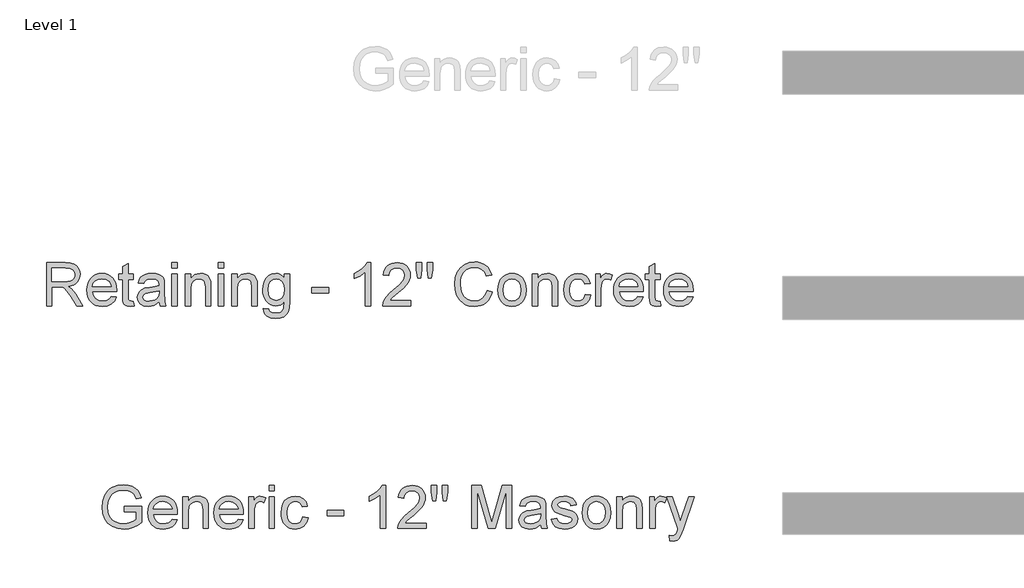
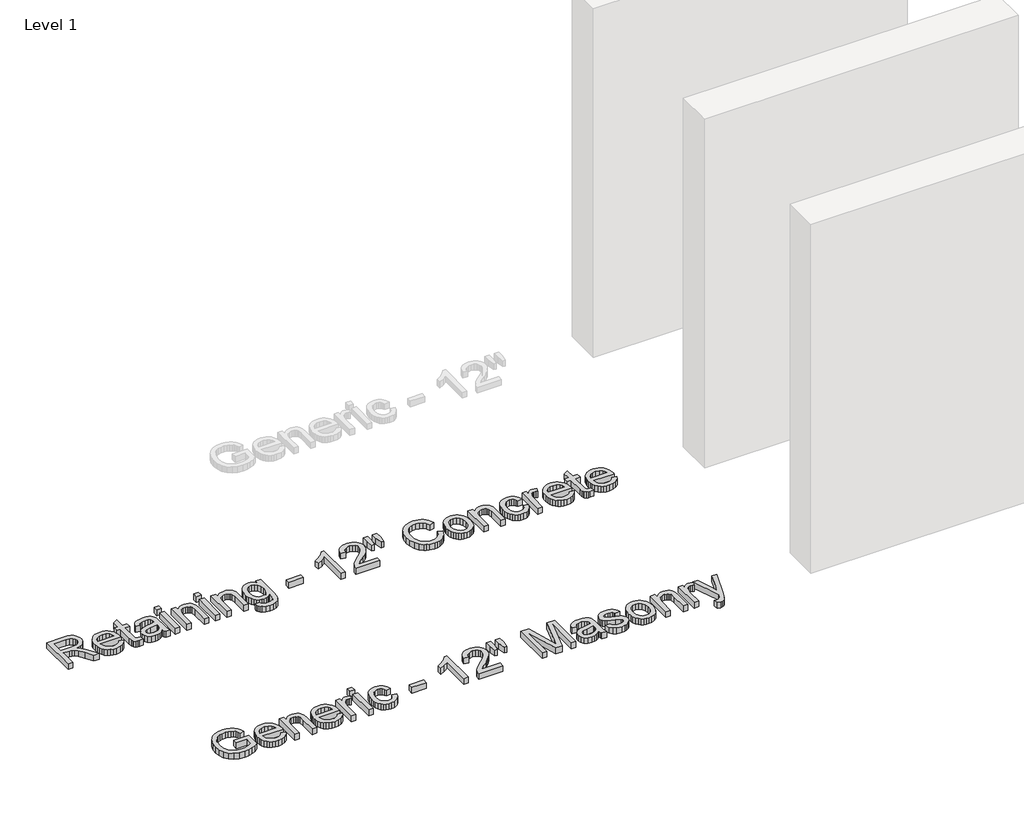
# One storey, part 19 of 42: 2 proxies.
"""IFC4 building model written with IfcOpenShell, lengths in millimetres."""

from ifc_helpers import new_model, si_unit, origin, origin_with_axes, place, context, project, spatial, polyline, outline, extrude, element, save

model = new_model("IFC4")

# Units and contexts
model_context = context("Model", 3, world=origin())
ifc_project = project(units=[si_unit("LENGTHUNIT", "METRE", prefix="MILLI")], contexts=[model_context])

# Site, building, storey
site = spatial("IfcSite", under=ifc_project)
building = spatial("IfcBuilding", under=site)
storey = spatial("IfcBuildingStorey", under=building, Name="Level 1", Elevation=0.0)

# Proxies
placement = place(None, origin())
element("IfcBuildingElementProxy", 1, Name="8\" Arial", ObjectType="8\" Arial", at=placement, inside=storey, context=model_context, shape_type="SweptSolid", body=[
    extrude(outline(polyline([(-17723.2374859, 6548.4833965), (-17723.2374859, 6853.0504905), (-17591.9970266, 6853.0504905), (-17556.7238295, 6850.9963729), (-17531.0613007, 6844.8340199), (-17512.3046968, 6833.4573682), (-17497.7492747, 6815.7603544), (-17488.4081514, 6793.8156855), (-17485.2944436, 6769.6960686), (-17490.4529744, 6739.6929381), (-17505.9285668, 6714.8204544), (-17517.6514442, 6704.6846385), (-17532.1859533, 6696.584351), (-17569.6898664, 6686.490361), (-17548.051921, 6670.206134), (-17517.1936827, 6631.0198893), (-17466.4077146, 6548.4833965), (-17510.6502491, 6548.4833965), (-17550.282637, 6611.6126599), (-17578.9101593, 6653.4014067), (-17599.0237821, 6673.1432435), (-17617.1297605, 6680.3930705), (-17639.2138491, 6681.7315001), (-17685.1665991, 6681.7315001), (-17685.1665991, 6548.4833965), (-17723.2374859, 6548.4833965)]), holes=[polyline([(-17685.1665991, 6719.8023869), (-17599.9532471, 6719.8023869), (-17575.4804334, 6721.1501112), (-17556.4914633, 6725.1932839), (-17542.1962915, 6732.2014501), (-17531.8048727, 6742.4441545), (-17525.4752159, 6754.8339231), (-17523.3653304, 6768.2832817), (-17527.3899139, 6786.8539926), (-17539.4636643, 6801.8183793), (-17560.2372073, 6811.6892977), (-17590.3611682, 6814.9796038), (-17685.1665991, 6814.9796038), (-17685.1665991, 6719.8023869)])]), origin_with_axes(), (0.0, 0.0, 1.0), 50.8),
    extrude(outline(polyline([(-17266.832988, 6615.1074483), (-17229.5056732, 6610.3485875), (-17242.9550319, 6582.2229763), (-17264.4163789, 6561.1984778), (-17293.4063926, 6548.0930212), (-17329.441751, 6543.7245356), (-17353.0641041, 6545.6090259), (-17374.1118393, 6551.2624969), (-17392.5849563, 6560.6849484), (-17408.4834553, 6573.8763805), (-17421.2682465, 6590.4696546), (-17430.4002402, 6610.0976319), (-17435.8794364, 6632.7603125), (-17437.7058352, 6658.4576963), (-17435.8608471, 6685.0264536), (-17430.325883, 6708.4443245), (-17421.1009428, 6728.711309), (-17408.1860265, 6745.8274071), (-17392.3293534, 6759.4254802), (-17374.279143, 6769.1383896), (-17354.0353951, 6774.9661352), (-17331.5981098, 6776.908717), (-17309.8834835, 6774.9707825), (-17290.2462115, 6769.1569789), (-17272.6862939, 6759.4673061), (-17257.2037305, 6745.9017643), (-17244.56533, 6728.8228448), (-17235.5379011, 6708.5930389), (-17230.1214438, 6685.2123466), (-17228.315958, 6658.6807679), (-17228.5390296, 6648.4194742), (-17399.6349484, 6648.4194742), (-17393.0450415, 6619.922077), (-17377.7367528, 6598.9719358), (-17355.6433695, 6586.0895507), (-17328.6981789, 6581.7954224), (-17308.4358418, 6583.7844775), (-17291.3708642, 6589.7516429), (-17277.5032463, 6600.0687045), (-17266.832988, 6615.1074483)]), holes=[polyline([(-17399.6349484, 6686.490361), (-17266.3868448, 6686.490361), (-17271.5360809, 6706.6039838), (-17281.6300709, 6720.9921021), (-17303.8256953, 6734.3763982), (-17331.7468242, 6738.8378303), (-17357.4093531, 6735.2779793), (-17378.6290392, 6724.5984263), (-17393.3796489, 6707.951708), (-17399.6349484, 6686.490361)])]), origin_with_axes(), (0.0, 0.0, 1.0), 50.8),
    extrude(outline(polyline([(-17109.3444369, 6580.2339212), (-17104.585576, 6547.3680385), (-17133.0643839, 6543.7245356), (-17151.337666, 6545.3046261), (-17164.963623, 6550.0448977), (-17174.5928805, 6557.3504927), (-17180.876064, 6566.6265534), (-17184.3336738, 6582.5575837), (-17185.4862104, 6609.8280871), (-17185.4862104, 6734.0789694), (-17214.0393755, 6734.0789694), (-17214.0393755, 6772.1498562), (-17185.4862104, 6772.1498562), (-17185.4862104, 6826.5049699), (-17147.4153236, 6848.8864873), (-17147.4153236, 6772.1498562), (-17109.3444369, 6772.1498562), (-17109.3444369, 6734.0789694), (-17147.4153236, 6734.0789694), (-17147.4153236, 6610.9434451), (-17145.4076792, 6591.3131441), (-17138.9014242, 6584.3607458), (-17125.9260926, 6581.7954224), (-17109.3444369, 6580.2339212)])), origin_with_axes(), (0.0, 0.0, 1.0), 50.8),
    extrude(outline(polyline([(-16928.5077248, 6577.0365615), (-16946.697355, 6561.4401387), (-16965.4260749, 6551.2346129), (-16985.1214385, 6545.602055), (-17006.2109995, 6543.7245356), (-17038.0265868, 6548.2417356), (-17061.4955782, 6561.7933354), (-17075.9673484, 6582.3716907), (-17080.7912718, 6607.969157), (-17078.9695204, 6623.7514729), (-17073.5042661, 6638.0838233), (-17065.0740185, 6650.3527614), (-17054.357287, 6659.9448403), (-17027.7002305, 6672.43685), (-16994.7599906, 6678.1623545), (-16955.833996, 6684.1852878), (-16928.7307964, 6691.2492218), (-16928.5077248, 6699.7259427), (-16931.1288161, 6716.7165631), (-16938.9920901, 6727.8329646), (-16956.577568, 6736.0866138), (-16981.0782657, 6738.8378303), (-17003.7572119, 6737.0067842), (-17019.5952956, 6731.513646), (-17030.395679, 6721.3545935), (-17037.9615242, 6705.5258044), (-17076.032411, 6710.2846652), (-17069.4239148, 6731.1046814), (-17059.562291, 6747.4632656), (-17045.5273694, 6759.9738646), (-17026.3989795, 6769.2499254), (-17003.0043452, 6774.9940191), (-16976.1706904, 6776.908717), (-16950.4338043, 6775.2170907), (-16930.0320474, 6770.1422118), (-16914.6494015, 6762.511304), (-16903.9698485, 6753.1515914), (-16896.8873252, 6741.579752), (-16892.295768, 6727.3124642), (-16890.436838, 6694.0004382), (-16890.436838, 6646.6349014), (-16888.5035508, 6580.4941714), (-16880.9191163, 6548.4833965), (-16918.9900031, 6548.4833965), (-16925.0872935, 6561.7189782), (-16928.5077248, 6577.0365615)]), holes=[polyline([(-16928.5077248, 6653.1783351), (-16989.9267726, 6641.5042546), (-17022.6811195, 6635.3326069), (-17037.515381, 6625.2943848), (-17042.7203851, 6610.6460163), (-17039.8855168, 6599.3251325), (-17031.3809119, 6590.0490717), (-17017.3924636, 6583.8588347), (-16998.1060646, 6581.7954224), (-16977.6578344, 6584.0726117), (-16959.5890347, 6590.9041795), (-16944.9406661, 6600.9702855), (-16934.7537296, 6612.9510895), (-16930.2365297, 6625.2943848), (-16928.7307964, 6642.396541), (-16928.5077248, 6653.1783351)])]), origin_with_axes(), (0.0, 0.0, 1.0), 50.8),
    extrude(outline(polyline([(-16838.0893687, 6814.9796038), (-16838.0893687, 6853.0504905), (-16800.018482, 6853.0504905), (-16800.018482, 6814.9796038), (-16838.0893687, 6814.9796038)])), origin_with_axes(), (0.0, 0.0, 1.0), 50.8),
    extrude(outline(polyline([(-16838.0893687, 6548.4833965), (-16838.0893687, 6772.1498562), (-16800.018482, 6772.1498562), (-16800.018482, 6548.4833965), (-16838.0893687, 6548.4833965)])), origin_with_axes(), (0.0, 0.0, 1.0), 50.8),
    extrude(outline(polyline([(-16742.9121518, 6548.4833965), (-16742.9121518, 6772.1498562), (-16704.8412651, 6772.1498562), (-16704.8412651, 6740.9198319), (-16691.614978, 6756.6649691), (-16675.730421, 6767.9114957), (-16657.1875941, 6774.6594117), (-16635.9864972, 6776.908717), (-16617.2205987, 6775.0962603), (-16600.0347907, 6769.65889), (-16585.7024402, 6761.2751156), (-16575.4969145, 6750.6234466), (-16564.0830841, 6722.6279605), (-16562.0754397, 6685.8211462), (-16562.0754397, 6548.4833965), (-16600.1463265, 6548.4833965), (-16600.1463265, 6680.6904993), (-16604.5334013, 6714.3743112), (-16610.6028078, 6724.4032387), (-16620.0368777, 6732.1828608), (-16632.1292174, 6737.1740879), (-16646.1734337, 6738.8378303), (-16668.4712993, 6735.1013809), (-16687.4788587, 6723.8920329), (-16695.0749115, 6714.7414499), (-16700.5006635, 6702.2354982), (-16704.8412651, 6667.1574888), (-16704.8412651, 6548.4833965), (-16742.9121518, 6548.4833965)])), origin_with_axes(), (0.0, 0.0, 1.0), 50.8),
    extrude(outline(polyline([(-16509.7279704, 6814.9796038), (-16509.7279704, 6853.0504905), (-16471.6570837, 6853.0504905), (-16471.6570837, 6814.9796038), (-16509.7279704, 6814.9796038)])), origin_with_axes(), (0.0, 0.0, 1.0), 50.8),
    extrude(outline(polyline([(-16509.7279704, 6548.4833965), (-16509.7279704, 6772.1498562), (-16471.6570837, 6772.1498562), (-16471.6570837, 6548.4833965), (-16509.7279704, 6548.4833965)])), origin_with_axes(), (0.0, 0.0, 1.0), 50.8),
    extrude(outline(polyline([(-16414.5507535, 6548.4833965), (-16414.5507535, 6772.1498562), (-16376.4798668, 6772.1498562), (-16376.4798668, 6740.9198319), (-16363.2535797, 6756.6649691), (-16347.3690227, 6767.9114957), (-16328.8261958, 6774.6594117), (-16307.6250989, 6776.908717), (-16288.8592004, 6775.0962603), (-16271.6733924, 6769.65889), (-16257.341042, 6761.2751156), (-16247.1355162, 6750.6234466), (-16235.7216859, 6722.6279605), (-16233.7140414, 6685.8211462), (-16233.7140414, 6548.4833965), (-16271.7849282, 6548.4833965), (-16271.7849282, 6680.6904993), (-16276.172003, 6714.3743112), (-16282.2414095, 6724.4032387), (-16291.6754794, 6732.1828608), (-16303.7678191, 6737.1740879), (-16317.8120354, 6738.8378303), (-16340.109901, 6735.1013809), (-16359.1174604, 6723.8920329), (-16366.7135132, 6714.7414499), (-16372.1392652, 6702.2354982), (-16376.4798668, 6667.1574888), (-16376.4798668, 6548.4833965), (-16414.5507535, 6548.4833965)])), origin_with_axes(), (0.0, 0.0, 1.0), 50.8),
    extrude(outline(polyline([(-16190.8842938, 6529.4479531), (-16152.8134071, 6524.6890923), (-16148.6122252, 6512.7919401), (-16140.4701118, 6504.6126481), (-16124.4647243, 6498.2551074), (-16103.514583, 6496.1359272), (-16081.1702442, 6498.5339469), (-16064.5514098, 6505.7280061), (-16053.0260437, 6517.2533722), (-16045.9621097, 6532.6453127), (-16043.3596076, 6577.0365615), (-16056.0282157, 6564.5445518), (-16070.1653785, 6555.6216877), (-16085.771096, 6550.2679693), (-16102.8453682, 6548.4833965), (-16123.7188286, 6550.5607508), (-16142.0966755, 6556.7928137), (-16157.9789089, 6567.1795851), (-16171.3655286, 6581.7210652), (-16181.98699, 6599.1671234), (-16189.5737482, 6618.2676293), (-16194.125803, 6639.022583), (-16195.6431547, 6661.4319843), (-16192.9198222, 6692.1693922), (-16184.7498248, 6720.4344231), (-16171.4212965, 6744.3867364), (-16153.2223717, 6762.1859913), (-16130.7757917, 6773.2280356), (-16104.7042982, 6776.908717), (-16086.900396, 6774.8267154), (-16070.7416468, 6768.5807106), (-16056.2280507, 6758.1707025), (-16043.3596076, 6743.5966911), (-16043.3596076, 6772.1498562), (-16005.2887209, 6772.1498562), (-16005.2887209, 6579.044206), (-16007.8912229, 6534.4577695), (-16015.698729, 6505.0959699), (-16029.1480877, 6485.6236779), (-16048.6761475, 6470.7057645), (-16073.8553546, 6461.2252215), (-16104.258155, 6458.0650404), (-16139.6800665, 6462.5171778), (-16167.5733114, 6475.87359), (-16178.0785897, 6485.9001938), (-16185.4655128, 6498.1714556), (-16189.7340809, 6512.6873753), (-16190.8842938, 6529.4479531)]), holes=[polyline([(-16157.5722679, 6664.0344864), (-16153.5105058, 6629.114486), (-16141.3252196, 6605.1064048), (-16123.0054642, 6591.1923136), (-16100.540295, 6586.5542832), (-16078.2424294, 6591.1644297), (-16059.8297276, 6604.994869), (-16047.4771376, 6628.6962267), (-16043.3596076, 6662.9191284), (-16047.5979681, 6695.9244308), (-16060.3130494, 6719.6908511), (-16078.9952961, 6734.0510855), (-16101.1351526, 6738.8378303), (-16122.8753391, 6734.1254427), (-16141.102148, 6719.9882799), (-16153.4547379, 6696.5750563), (-16157.5722679, 6664.0344864)])]), origin_with_axes(), (0.0, 0.0, 1.0), 50.8),
    extrude(outline(polyline([(-15848.246313, 6638.9017525), (-15848.246313, 6676.9726393), (-15729.2747919, 6676.9726393), (-15729.2747919, 6638.9017525), (-15848.246313, 6638.9017525)])), origin_with_axes(), (0.0, 0.0, 1.0), 50.8),
    extrude(outline(polyline([(-15434.2254195, 6548.4833965), (-15472.2963063, 6548.4833965), (-15472.2963063, 6785.8315811), (-15508.3595486, 6760.1411683), (-15548.4380798, 6740.9198319), (-15548.4380798, 6776.908717), (-15518.5371904, 6793.1743547), (-15492.6330007, 6812.5258162), (-15472.2126544, 6833.1041715), (-15458.7632957, 6853.0504905), (-15434.2254195, 6853.0504905), (-15434.2254195, 6548.4833965)])), origin_with_axes(), (0.0, 0.0, 1.0), 50.8),
    extrude(outline(polyline([(-15148.6937688, 6586.5542832), (-15148.6937688, 6548.4833965), (-15348.5659243, 6548.4833965), (-15344.4762783, 6574.7314883), (-15335.0886817, 6595.2447811), (-15321.3511888, 6615.1446269), (-15301.479227, 6635.9739378), (-15273.6882232, 6659.2756255), (-15232.6058698, 6695.7664218), (-15207.9564578, 6722.7023177), (-15195.6317518, 6744.5633347), (-15191.5235164, 6765.8294941), (-15195.3993855, 6784.8928215), (-15207.0269928, 6800.7401999), (-15224.9006049, 6811.4197528), (-15247.5144885, 6814.9796038), (-15271.2623195, 6811.5034047), (-15289.7121999, 6801.0748073), (-15301.6186467, 6784.5117408), (-15305.7361767, 6762.6321345), (-15343.8070635, 6767.3909953), (-15340.533023, 6787.0445329), (-15334.5774759, 6804.216399), (-15325.9404223, 6818.9065934), (-15314.6218622, 6831.1151163), (-15300.8820457, 6840.7118426), (-15284.981223, 6847.566647), (-15246.6965593, 6853.0504905), (-15226.2924787, 6851.5261679), (-15208.1330561, 6846.9532001), (-15192.2182915, 6839.331587), (-15178.5481849, 6828.6613287), (-15167.5688795, 6815.7324704), (-15159.7265185, 6801.3350575), (-15155.0211019, 6785.4690898), (-15153.4526297, 6768.1345673), (-15155.144256, 6749.9263478), (-15160.2191349, 6732.0341464), (-15169.2256509, 6713.8352215), (-15182.7121881, 6694.7068317), (-15204.2107138, 6671.8698764), (-15237.2531948, 6642.5452554), (-15281.0495861, 6605.924334), (-15298.2260994, 6586.5542832), (-15148.6937688, 6586.5542832)])), origin_with_axes(), (0.0, 0.0, 1.0), 50.8),
    extrude(outline(polyline([(-15101.328232, 6743.5966911), (-15110.6228821, 6802.4132369), (-15110.6228821, 6853.0504905), (-15072.5519953, 6853.0504905), (-15072.5519953, 6802.4132369), (-15080.8800018, 6743.5966911), (-15101.328232, 6743.5966911)])), origin_with_axes(), (0.0, 0.0, 1.0), 50.8),
    extrude(outline(polyline([(-15025.4095301, 6743.5966911), (-15034.4811085, 6802.4132369), (-15034.4811085, 6853.0504905), (-14996.4102218, 6853.0504905), (-14996.4102218, 6802.4132369), (-15005.3330859, 6743.5966911), (-15025.4095301, 6743.5966911)])), origin_with_axes(), (0.0, 0.0, 1.0), 50.8),
    extrude(outline(polyline([(-14610.9424933, 6656.7474807), (-14572.8716066, 6646.9323302), (-14580.4049205, 6623.2565328), (-14590.4384953, 6602.5689653), (-14602.9723309, 6584.8696279), (-14618.0064274, 6570.1585205), (-14635.2015301, 6558.5936521), (-14654.2183842, 6550.3330318), (-14675.0569897, 6545.3766597), (-14697.7173466, 6543.7245356), (-14741.8762291, 6548.7250574), (-14760.5468575, 6554.9757096), (-14776.9449439, 6563.7266226), (-14803.825072, 6588.208731), (-14823.4181944, 6621.650882), (-14835.380409, 6660.9672518), (-14839.3678139, 6703.0720167), (-14834.8599086, 6747.4818549), (-14821.3361927, 6785.8315811), (-14799.5030597, 6816.9035964), (-14770.0669028, 6839.4803014), (-14735.1561971, 6853.2270889), (-14696.8994174, 6857.8093514), (-14675.1243759, 6856.3268547), (-14655.1571438, 6851.8793646), (-14636.9977212, 6844.4668812), (-14620.646108, 6834.0894044), (-14606.3718492, 6821.0211263), (-14594.4444894, 6805.5362393), (-14577.6304674, 6767.3166381), (-14615.7013542, 6758.2450597), (-14628.8997573, 6786.0081795), (-14646.9313785, 6805.0529175), (-14670.0192893, 6816.0670778), (-14698.3865614, 6819.7384646), (-14731.0851404, 6815.6674079), (-14757.9466791, 6803.4542377), (-14778.3298468, 6784.3816157), (-14791.5933125, 6759.7322037), (-14798.8710235, 6731.8668427), (-14801.2969271, 6703.1463739), (-14798.4248803, 6667.975418), (-14789.8087396, 6637.5633229), (-14775.1231925, 6613.0719199), (-14754.0429261, 6595.6630403), (-14728.7707725, 6585.2623269), (-14701.5095638, 6581.7954224), (-14669.7311552, 6586.5171046), (-14643.2506971, 6600.6821514), (-14623.2579047, 6624.1418482), (-14610.9424933, 6656.7474807)])), origin_with_axes(), (0.0, 0.0, 1.0), 50.8),
    extrude(outline(polyline([(-14534.8007198, 6660.3166263), (-14532.7419548, 6689.2834033), (-14526.5656599, 6714.2441861), (-14516.2718349, 6735.1989748), (-14501.8604799, 6752.1477692), (-14487.3515311, 6762.9806839), (-14471.336849, 6770.7184801), (-14453.8164336, 6775.3611578), (-14434.7902849, 6776.908717), (-14413.7866994, 6775.0242267), (-14394.7954056, 6769.3707558), (-14377.8164035, 6759.9483043), (-14362.8496932, 6746.7568721), (-14350.6341993, 6730.2426026), (-14341.9088466, 6710.8516389), (-14336.6736349, 6688.5839809), (-14334.9285644, 6663.4396288), (-14338.0143882, 6624.9783667), (-14347.2718597, 6595.7002189), (-14362.431434, 6573.7741394), (-14383.2235662, 6557.369082), (-14407.9194515, 6547.1356722), (-14434.7902849, 6543.7245356), (-14456.1005939, 6545.602055), (-14475.268486, 6551.2346129), (-14492.2939613, 6560.6222095), (-14507.1770198, 6573.7648447), (-14519.2623885, 6590.439447), (-14527.8947948, 6610.4229447), (-14533.0742386, 6633.7153378), (-14534.8007198, 6660.3166263)]), holes=[polyline([(-14496.7298331, 6660.3909835), (-14492.3241689, 6625.9357157), (-14479.1071765, 6601.3885448), (-14459.2166253, 6586.693703), (-14434.7902849, 6581.7954224), (-14410.4754803, 6586.7215869), (-14390.6221077, 6601.5000806), (-14377.4051153, 6626.3725642), (-14372.9994511, 6661.5806987), (-14377.4329992, 6695.0321444), (-14390.7336435, 6719.2447079), (-14410.6149, 6733.9395497), (-14434.7902849, 6738.8378303), (-14459.2166253, 6733.958139), (-14479.1071765, 6719.3190651), (-14492.3241689, 6694.8276621), (-14496.7298331, 6660.3909835)])]), origin_with_axes(), (0.0, 0.0, 1.0), 50.8),
    extrude(outline(polyline([(-14292.0988167, 6548.4833965), (-14292.0988167, 6772.1498562), (-14254.02793, 6772.1498562), (-14254.02793, 6740.9198319), (-14240.8016429, 6756.6649691), (-14224.9170859, 6767.9114957), (-14206.374259, 6774.6594117), (-14185.1731621, 6776.908717), (-14166.4072636, 6775.0962603), (-14149.2214556, 6769.65889), (-14134.8891052, 6761.2751156), (-14124.6835794, 6750.6234466), (-14113.2697491, 6722.6279605), (-14111.2621046, 6685.8211462), (-14111.2621046, 6548.4833965), (-14149.3329914, 6548.4833965), (-14149.3329914, 6680.6904993), (-14153.7200662, 6714.3743112), (-14159.7894728, 6724.4032387), (-14169.2235426, 6732.1828608), (-14181.3158824, 6737.1740879), (-14195.3600986, 6738.8378303), (-14217.6579642, 6735.1013809), (-14236.6655236, 6723.8920329), (-14244.2615764, 6714.7414499), (-14249.6873284, 6702.2354982), (-14254.02793, 6667.1574888), (-14254.02793, 6548.4833965), (-14292.0988167, 6548.4833965)])), origin_with_axes(), (0.0, 0.0, 1.0), 50.8),
    extrude(outline(polyline([(-13916.14881, 6629.3840308), (-13878.0779232, 6624.62517), (-13888.6924136, 6590.7647597), (-13908.6387327, 6565.176588), (-13936.0393612, 6549.0875487), (-13969.0167797, 6543.7245356), (-13990.3689146, 6545.595084), (-14009.5135701, 6551.206729), (-14026.4507463, 6560.5594706), (-14041.180443, 6573.6533089), (-14053.1031554, 6590.2419357), (-14061.6193785, 6610.0790426), (-14066.7291124, 6633.1646298), (-14068.432357, 6659.4986971), (-14065.5231316, 6693.3776967), (-14056.7954551, 6722.7394963), (-14042.109908, 6746.4501487), (-14021.3270704, 6763.3757065), (-13996.4638814, 6773.5254644), (-13969.5372801, 6776.908717), (-13937.3684962, 6772.261392), (-13911.6501994, 6758.3194169), (-13893.2003189, 6735.8263636), (-13882.8367841, 6705.5258044), (-13920.9076709, 6700.7669435), (-13927.8135959, 6717.3764832), (-13938.567506, 6729.28293), (-13952.5745437, 6736.4491052), (-13969.2398513, 6738.8378303), (-13993.8427901, 6734.1347373), (-14013.3708499, 6720.0254585), (-14026.1138152, 6695.7478325), (-14030.3614703, 6660.5396979), (-14026.2067617, 6624.8575362), (-14013.7426359, 6600.4962584), (-13994.5677728, 6586.4706314), (-13970.2808521, 6581.7954224), (-13950.5668993, 6584.7139425), (-13934.4035028, 6593.4695029), (-13922.6457704, 6608.2851751), (-13916.14881, 6629.3840308)])), origin_with_axes(), (0.0, 0.0, 1.0), 50.8),
    extrude(outline(polyline([(-13844.7658973, 6548.4833965), (-13844.7658973, 6772.1498562), (-13811.4538714, 6772.1498562), (-13811.4538714, 6739.0609019), (-13799.1477547, 6758.2450597), (-13787.8082816, 6769.5473542), (-13776.4316299, 6775.0683763), (-13764.0139774, 6776.908717), (-13745.0528912, 6773.9716076), (-13725.7943762, 6765.1602793), (-13738.5094575, 6731.0303242), (-13751.8937537, 6736.8859538), (-13765.2780498, 6738.8378303), (-13776.6454068, 6736.960311), (-13786.8044594, 6731.327753), (-13795.0116354, 6722.3677103), (-13800.5233629, 6710.5077368), (-13805.1520987, 6689.2415774), (-13806.6950106, 6666.0421308), (-13806.6950106, 6548.4833965), (-13844.7658973, 6548.4833965)])), origin_with_axes(), (0.0, 0.0, 1.0), 50.8),
    extrude(outline(polyline([(-13545.4038073, 6615.1074483), (-13508.0764926, 6610.3485875), (-13521.5258512, 6582.2229763), (-13542.9871983, 6561.1984778), (-13571.9772119, 6548.0930212), (-13608.0125703, 6543.7245356), (-13631.6349235, 6545.6090259), (-13652.6826586, 6551.2624969), (-13671.1557757, 6560.6849484), (-13687.0542746, 6573.8763805), (-13699.8390658, 6590.4696546), (-13708.9710596, 6610.0976319), (-13714.4502558, 6632.7603125), (-13716.2766545, 6658.4576963), (-13714.4316665, 6685.0264536), (-13708.8967024, 6708.4443245), (-13699.6717621, 6728.711309), (-13686.7568458, 6745.8274071), (-13670.9001728, 6759.4254802), (-13652.8499623, 6769.1383896), (-13632.6062144, 6774.9661352), (-13610.1689291, 6776.908717), (-13588.4543029, 6774.9707825), (-13568.8170309, 6769.1569789), (-13551.2571132, 6759.4673061), (-13535.7745498, 6745.9017643), (-13523.1361494, 6728.8228448), (-13514.1087205, 6708.5930389), (-13508.6922631, 6685.2123466), (-13506.8867774, 6658.6807679), (-13507.109849, 6648.4194742), (-13678.2057678, 6648.4194742), (-13671.6158609, 6619.922077), (-13656.3075722, 6598.9719358), (-13634.2141889, 6586.0895507), (-13607.2689983, 6581.7954224), (-13587.0066611, 6583.7844775), (-13569.9416835, 6589.7516429), (-13556.0740656, 6600.0687045), (-13545.4038073, 6615.1074483)]), holes=[polyline([(-13678.2057678, 6686.490361), (-13544.9576641, 6686.490361), (-13550.1069003, 6706.6039838), (-13560.2008903, 6720.9921021), (-13582.3965147, 6734.3763982), (-13610.3176435, 6738.8378303), (-13635.9801724, 6735.2779793), (-13657.1998586, 6724.5984263), (-13671.9504683, 6707.951708), (-13678.2057678, 6686.490361)])]), origin_with_axes(), (0.0, 0.0, 1.0), 50.8),
    extrude(outline(polyline([(-13387.9152562, 6580.2339212), (-13383.1563954, 6547.3680385), (-13411.6352033, 6543.7245356), (-13429.9084853, 6545.3046261), (-13443.5344424, 6550.0448977), (-13453.1636998, 6557.3504927), (-13459.4468833, 6566.6265534), (-13462.9044931, 6582.5575837), (-13464.0570297, 6609.8280871), (-13464.0570297, 6734.0789694), (-13492.6101948, 6734.0789694), (-13492.6101948, 6772.1498562), (-13464.0570297, 6772.1498562), (-13464.0570297, 6826.5049699), (-13425.986143, 6848.8864873), (-13425.986143, 6772.1498562), (-13387.9152562, 6772.1498562), (-13387.9152562, 6734.0789694), (-13425.986143, 6734.0789694), (-13425.986143, 6610.9434451), (-13423.9784986, 6591.3131441), (-13417.4722435, 6584.3607458), (-13404.496912, 6581.7954224), (-13387.9152562, 6580.2339212)])), origin_with_axes(), (0.0, 0.0, 1.0), 50.8),
    extrude(outline(polyline([(-13193.2481048, 6615.1074483), (-13155.92079, 6610.3485875), (-13169.3701487, 6582.2229763), (-13190.8314958, 6561.1984778), (-13219.8215094, 6548.0930212), (-13255.8568678, 6543.7245356), (-13279.479221, 6545.6090259), (-13300.5269561, 6551.2624969), (-13319.0000732, 6560.6849484), (-13334.8985721, 6573.8763805), (-13347.6833633, 6590.4696546), (-13356.815357, 6610.0976319), (-13362.2945533, 6632.7603125), (-13364.120952, 6658.4576963), (-13362.275964, 6685.0264536), (-13356.7409998, 6708.4443245), (-13347.5160596, 6728.711309), (-13334.6011433, 6745.8274071), (-13318.7444703, 6759.4254802), (-13300.6942598, 6769.1383896), (-13280.4505119, 6774.9661352), (-13258.0132266, 6776.908717), (-13236.2986003, 6774.9707825), (-13216.6613284, 6769.1569789), (-13199.1014107, 6759.4673061), (-13183.6188473, 6745.9017643), (-13170.9804469, 6728.8228448), (-13161.953018, 6708.5930389), (-13156.5365606, 6685.2123466), (-13154.7310748, 6658.6807679), (-13154.9541464, 6648.4194742), (-13326.0500652, 6648.4194742), (-13319.4601583, 6619.922077), (-13304.1518696, 6598.9719358), (-13282.0584864, 6586.0895507), (-13255.1132958, 6581.7954224), (-13234.8509586, 6583.7844775), (-13217.785981, 6589.7516429), (-13203.9183631, 6600.0687045), (-13193.2481048, 6615.1074483)]), holes=[polyline([(-13326.0500652, 6686.490361), (-13192.8019616, 6686.490361), (-13197.9511977, 6706.6039838), (-13208.0451877, 6720.9921021), (-13230.2408121, 6734.3763982), (-13258.161941, 6738.8378303), (-13283.8244699, 6735.2779793), (-13305.0441561, 6724.5984263), (-13319.7947657, 6707.951708), (-13326.0500652, 6686.490361)])]), origin_with_axes(), (0.0, 0.0, 1.0), 50.8),
])
element("IfcBuildingElementProxy", 2, Name="8\" Arial", ObjectType="8\" Arial", at=placement, inside=storey, context=model_context, shape_type="SweptSolid", body=[
    extrude(outline(polyline([(-17174.0716605, 5092.6549176), (-17174.0716605, 5130.7258044), (-17050.3412786, 5130.7258044), (-17050.3412786, 5016.8849301), (-17080.4094716, 4995.9719674), (-17111.4257189, 4980.9704021), (-17143.3156634, 4971.9360023), (-17176.0049477, 4968.9245356), (-17218.7138649, 4973.7112804), (-17257.3145467, 4988.0715148), (-17289.3810895, 5011.5033277), (-17312.4875896, 5043.5048079), (-17326.4574487, 5081.8917128), (-17331.1140684, 5124.4797995), (-17326.476038, 5167.3746097), (-17312.5619468, 5207.2765425), (-17289.9480632, 5240.7465774), (-17275.5947998, 5253.7800005), (-17259.2106553, 5264.345694), (-17221.7718048, 5278.343437), (-17179.053593, 5283.0093514), (-17147.6934436, 5280.3046082), (-17119.4934752, 5272.1903787), (-17095.7456442, 5259.2522258), (-17077.741907, 5242.0757124), (-17064.4226734, 5219.8336147), (-17054.7283534, 5191.6987089), (-17089.8249521, 5181.8092012), (-17097.6603421, 5201.8763508), (-17107.1873585, 5217.0173358), (-17119.790904, 5228.4311661), (-17136.8558816, 5237.3168516), (-17157.2018706, 5243.0330614), (-17179.6484506, 5244.9384646), (-17205.9244264, 5242.884347), (-17228.3895956, 5236.721994), (-17246.9603065, 5227.2228616), (-17261.5529071, 5215.1584058), (-17281.1460295, 5185.8244901), (-17290.0688936, 5157.085432), (-17293.0431816, 5126.0413007), (-17289.4647414, 5089.6341563), (-17278.7294205, 5059.6774991), (-17261.1625318, 5036.385106), (-17237.0893881, 5019.9707539), (-17208.9173037, 5010.2392553), (-17179.053593, 5006.9954224), (-17152.6846707, 5009.4399154), (-17126.9663739, 5016.7733943), (-17104.6313297, 5026.8766789), (-17088.4121653, 5037.6305891), (-17088.4121653, 5092.6549176), (-17174.0716605, 5092.6549176)])), origin_with_axes(), (0.0, 0.0, 1.0), 50.8),
    extrude(outline(polyline([(-16836.6386837, 5040.3074483), (-16799.311369, 5035.5485875), (-16812.7607277, 5007.4229763), (-16834.2220747, 4986.3984778), (-16863.2120883, 4973.2930212), (-16899.2474467, 4968.9245356), (-16922.8697999, 4970.8090259), (-16943.917535, 4976.4624969), (-16962.3906521, 4985.8849484), (-16978.2891511, 4999.0763805), (-16991.0739423, 5015.6696546), (-17000.205936, 5035.2976319), (-17005.6851322, 5057.9603125), (-17007.5115309, 5083.6576963), (-17005.6665429, 5110.2264536), (-17000.1315788, 5133.6443245), (-16990.9066386, 5153.911309), (-16977.9917223, 5171.0274071), (-16962.1350492, 5184.6254802), (-16944.0848387, 5194.3383896), (-16923.8410909, 5200.1661352), (-16901.4038055, 5202.108717), (-16879.6891793, 5200.1707825), (-16860.0519073, 5194.3569789), (-16842.4919896, 5184.6673061), (-16827.0094262, 5171.1017643), (-16814.3710258, 5154.0228448), (-16805.3435969, 5133.7930389), (-16799.9271396, 5110.4123466), (-16798.1216538, 5083.8807679), (-16798.3447254, 5073.6194742), (-16969.4406442, 5073.6194742), (-16962.8507373, 5045.122077), (-16947.5424486, 5024.1719358), (-16925.4490653, 5011.2895507), (-16898.5038747, 5006.9954224), (-16878.2415375, 5008.9844775), (-16861.17656, 5014.9516429), (-16847.308942, 5025.2687045), (-16836.6386837, 5040.3074483)]), holes=[polyline([(-16969.4406442, 5111.690361), (-16836.1925405, 5111.690361), (-16841.3417767, 5131.8039838), (-16851.4357667, 5146.1921021), (-16873.6313911, 5159.5763982), (-16901.5525199, 5164.0378303), (-16927.2150488, 5160.4779793), (-16948.434735, 5149.7984263), (-16963.1853447, 5133.151708), (-16969.4406442, 5111.690361)])]), origin_with_axes(), (0.0, 0.0, 1.0), 50.8),
    extrude(outline(polyline([(-16760.050767, 4973.6833965), (-16760.050767, 5197.3498562), (-16721.9798803, 5197.3498562), (-16721.9798803, 5166.1198319), (-16708.7535932, 5181.8649691), (-16692.8690362, 5193.1114957), (-16674.3262093, 5199.8594117), (-16653.1251124, 5202.108717), (-16634.3592139, 5200.2962603), (-16617.1734059, 5194.85889), (-16602.8410554, 5186.4751156), (-16592.6355296, 5175.8234466), (-16581.2216993, 5147.8279605), (-16579.2140549, 5111.0211462), (-16579.2140549, 4973.6833965), (-16617.2849417, 4973.6833965), (-16617.2849417, 5105.8904993), (-16621.6720165, 5139.5743112), (-16627.741423, 5149.6032387), (-16637.1754929, 5157.3828608), (-16649.2678326, 5162.3740879), (-16663.3120489, 5164.0378303), (-16685.6099145, 5160.3013809), (-16704.6174739, 5149.0920329), (-16712.2135267, 5139.9414499), (-16717.6392787, 5127.4354982), (-16721.9798803, 5092.3574888), (-16721.9798803, 4973.6833965), (-16760.050767, 4973.6833965)])), origin_with_axes(), (0.0, 0.0, 1.0), 50.8),
    extrude(outline(polyline([(-16370.2703209, 5040.3074483), (-16332.9430062, 5035.5485875), (-16346.3923649, 5007.4229763), (-16367.8537119, 4986.3984778), (-16396.8437255, 4973.2930212), (-16432.8790839, 4968.9245356), (-16456.5014371, 4970.8090259), (-16477.5491723, 4976.4624969), (-16496.0222893, 4985.8849484), (-16511.9207883, 4999.0763805), (-16524.7055795, 5015.6696546), (-16533.8375732, 5035.2976319), (-16539.3167694, 5057.9603125), (-16541.1431682, 5083.6576963), (-16539.2981801, 5110.2264536), (-16533.763216, 5133.6443245), (-16524.5382758, 5153.911309), (-16511.6233595, 5171.0274071), (-16495.7666864, 5184.6254802), (-16477.716476, 5194.3383896), (-16457.4727281, 5200.1661352), (-16435.0354428, 5202.108717), (-16413.3208165, 5200.1707825), (-16393.6835445, 5194.3569789), (-16376.1236268, 5184.6673061), (-16360.6410635, 5171.1017643), (-16348.002663, 5154.0228448), (-16338.9752341, 5133.7930389), (-16333.5587768, 5110.4123466), (-16331.753291, 5083.8807679), (-16331.9763626, 5073.6194742), (-16503.0722814, 5073.6194742), (-16496.4823745, 5045.122077), (-16481.1740858, 5024.1719358), (-16459.0807025, 5011.2895507), (-16432.1355119, 5006.9954224), (-16411.8731747, 5008.9844775), (-16394.8081972, 5014.9516429), (-16380.9405792, 5025.2687045), (-16370.2703209, 5040.3074483)]), holes=[polyline([(-16503.0722814, 5111.690361), (-16369.8241777, 5111.690361), (-16374.9734139, 5131.8039838), (-16385.0674039, 5146.1921021), (-16407.2630283, 5159.5763982), (-16435.1841572, 5164.0378303), (-16460.846686, 5160.4779793), (-16482.0663722, 5149.7984263), (-16496.8169819, 5133.151708), (-16503.0722814, 5111.690361)])]), origin_with_axes(), (0.0, 0.0, 1.0), 50.8),
    extrude(outline(polyline([(-16293.6824042, 4973.6833965), (-16293.6824042, 5197.3498562), (-16260.3703783, 5197.3498562), (-16260.3703783, 5164.2609019), (-16248.0642616, 5183.4450597), (-16236.7247885, 5194.7473542), (-16225.3481368, 5200.2683763), (-16212.9304843, 5202.108717), (-16193.9693981, 5199.1716076), (-16174.7108831, 5190.3602793), (-16187.4259644, 5156.2303242), (-16200.8102605, 5162.0859538), (-16214.1945567, 5164.0378303), (-16225.5619137, 5162.160311), (-16235.7209663, 5156.527753), (-16243.9281423, 5147.5677103), (-16249.4398698, 5135.7077368), (-16254.0686056, 5114.4415774), (-16255.6115175, 5091.2421308), (-16255.6115175, 4973.6833965), (-16293.6824042, 4973.6833965)])), origin_with_axes(), (0.0, 0.0, 1.0), 50.8),
    extrude(outline(polyline([(-16150.9165789, 5240.1796038), (-16150.9165789, 5278.2504905), (-16112.8456921, 5278.2504905), (-16112.8456921, 5240.1796038), (-16150.9165789, 5240.1796038)])), origin_with_axes(), (0.0, 0.0, 1.0), 50.8),
    extrude(outline(polyline([(-16150.9165789, 4973.6833965), (-16150.9165789, 5197.3498562), (-16112.8456921, 5197.3498562), (-16112.8456921, 4973.6833965), (-16150.9165789, 4973.6833965)])), origin_with_axes(), (0.0, 0.0, 1.0), 50.8),
    extrude(outline(polyline([(-15912.9735366, 5054.5840308), (-15874.9026499, 5049.82517), (-15885.5171403, 5015.9647597), (-15905.4634594, 4990.376588), (-15932.8640878, 4974.2875487), (-15965.8415063, 4968.9245356), (-15987.1936413, 4970.795084), (-16006.3382968, 4976.406729), (-16023.2754729, 4985.7594706), (-16038.0051696, 4998.8533089), (-16049.927882, 5015.4419357), (-16058.4441052, 5035.2790426), (-16063.553839, 5058.3646298), (-16065.2570837, 5084.6986971), (-16062.3478582, 5118.5776967), (-16053.6201818, 5147.9394963), (-16038.9346346, 5171.6501487), (-16018.151797, 5188.5757065), (-15993.288608, 5198.7254644), (-15966.3620067, 5202.108717), (-15934.1932228, 5197.461392), (-15908.474926, 5183.5194169), (-15890.0250456, 5161.0263636), (-15879.6615107, 5130.7258044), (-15917.7323975, 5125.9669435), (-15924.6383225, 5142.5764832), (-15935.3922327, 5154.48293), (-15949.3992703, 5161.6491052), (-15966.0645779, 5164.0378303), (-15990.6675167, 5159.3347373), (-16010.1955766, 5145.2254585), (-16022.9385418, 5120.9478325), (-16027.1861969, 5085.7396979), (-16023.0314883, 5050.0575362), (-16010.5673626, 5025.6962584), (-15991.3924994, 5011.6706314), (-15967.1055787, 5006.9954224), (-15947.3916259, 5009.9139425), (-15931.2282294, 5018.6695029), (-15919.4704971, 5033.4851751), (-15912.9735366, 5054.5840308)])), origin_with_axes(), (0.0, 0.0, 1.0), 50.8),
    extrude(outline(polyline([(-15741.6545462, 5064.1017525), (-15741.6545462, 5102.1726393), (-15622.6830251, 5102.1726393), (-15622.6830251, 5064.1017525), (-15741.6545462, 5064.1017525)])), origin_with_axes(), (0.0, 0.0, 1.0), 50.8),
    extrude(outline(polyline([(-15327.6336527, 4973.6833965), (-15365.7045395, 4973.6833965), (-15365.7045395, 5211.0315811), (-15401.7677818, 5185.3411683), (-15441.846313, 5166.1198319), (-15441.846313, 5202.108717), (-15411.9454237, 5218.3743547), (-15386.0412339, 5237.7258162), (-15365.6208876, 5258.3041715), (-15352.171529, 5278.2504905), (-15327.6336527, 5278.2504905), (-15327.6336527, 4973.6833965)])), origin_with_axes(), (0.0, 0.0, 1.0), 50.8),
    extrude(outline(polyline([(-15042.102002, 5011.7542832), (-15042.102002, 4973.6833965), (-15241.9741575, 4973.6833965), (-15237.8845115, 4999.9314883), (-15228.4969149, 5020.4447811), (-15214.7594221, 5040.3446269), (-15194.8874602, 5061.1739378), (-15167.0964564, 5084.4756255), (-15126.014103, 5120.9664218), (-15101.364691, 5147.9023177), (-15089.039985, 5169.7633347), (-15084.9317496, 5191.0294941), (-15088.8076187, 5210.0928215), (-15100.435226, 5225.9401999), (-15118.3088381, 5236.6197528), (-15140.9227218, 5240.1796038), (-15164.6705527, 5236.7034047), (-15183.1204332, 5226.2748073), (-15195.0268799, 5209.7117408), (-15199.1444099, 5187.8321345), (-15237.2152967, 5192.5909953), (-15233.9412562, 5212.2445329), (-15227.9857091, 5229.416399), (-15219.3486555, 5244.1065934), (-15208.0300954, 5256.3151163), (-15194.2902789, 5265.9118426), (-15178.3894563, 5272.766647), (-15140.1047926, 5278.2504905), (-15119.700712, 5276.7261679), (-15101.5412893, 5272.1532001), (-15085.6265247, 5264.531587), (-15071.9564181, 5253.8613287), (-15060.9771127, 5240.9324704), (-15053.1347517, 5226.5350575), (-15048.4293351, 5210.6690898), (-15046.8608629, 5193.3345673), (-15048.5524892, 5175.1263478), (-15053.6273681, 5157.2341464), (-15062.6338841, 5139.0352215), (-15076.1204214, 5119.9068317), (-15097.618947, 5097.0698764), (-15130.6614281, 5067.7452554), (-15174.4578193, 5031.124334), (-15191.6343326, 5011.7542832), (-15042.102002, 5011.7542832)])), origin_with_axes(), (0.0, 0.0, 1.0), 50.8),
    extrude(outline(polyline([(-14994.7364652, 5168.7966911), (-15004.0311153, 5227.6132369), (-15004.0311153, 5278.2504905), (-14965.9602285, 5278.2504905), (-14965.9602285, 5227.6132369), (-14974.288235, 5168.7966911), (-14994.7364652, 5168.7966911)])), origin_with_axes(), (0.0, 0.0, 1.0), 50.8),
    extrude(outline(polyline([(-14918.8177633, 5168.7966911), (-14927.8893418, 5227.6132369), (-14927.8893418, 5278.2504905), (-14889.818455, 5278.2504905), (-14889.818455, 5227.6132369), (-14898.7413191, 5168.7966911), (-14918.8177633, 5168.7966911)])), origin_with_axes(), (0.0, 0.0, 1.0), 50.8),
    extrude(outline(polyline([(-14718.4994646, 4973.6833965), (-14718.4994646, 5278.2504905), (-14652.9907708, 5278.2504905), (-14590.6794366, 5063.5812521), (-14578.1130697, 5018.7438601), (-14564.5057019, 5067.2991122), (-14503.2353686, 5278.2504905), (-14437.7266747, 5278.2504905), (-14437.7266747, 4973.6833965), (-14475.7975615, 4973.6833965), (-14475.7975615, 5240.1796038), (-14552.311121, 4973.6833965), (-14603.9150183, 4973.6833965), (-14680.4285778, 5240.1796038), (-14680.4285778, 4973.6833965), (-14718.4994646, 4973.6833965)])), origin_with_axes(), (0.0, 0.0, 1.0), 50.8),
    extrude(outline(polyline([(-14233.0956584, 5002.2365615), (-14251.2852886, 4986.6401387), (-14270.0140086, 4976.4346129), (-14289.7093721, 4970.802055), (-14310.7989332, 4968.9245356), (-14342.6145204, 4973.4417356), (-14366.0835119, 4986.9933354), (-14380.5552821, 5007.5716907), (-14385.3792055, 5033.169157), (-14383.557454, 5048.9514729), (-14378.0921998, 5063.2838233), (-14369.6619522, 5075.5527614), (-14358.9452206, 5085.1448403), (-14332.2881642, 5097.63685), (-14299.3479242, 5103.3623545), (-14260.4219297, 5109.3852878), (-14233.31873, 5116.4492218), (-14233.0956584, 5124.9259427), (-14235.7167497, 5141.9165631), (-14243.5800237, 5153.0329646), (-14261.1655017, 5161.2866138), (-14285.6661993, 5164.0378303), (-14308.3451455, 5162.2067842), (-14324.1832293, 5156.713646), (-14334.9836127, 5146.5545935), (-14342.5494578, 5130.7258044), (-14380.6203446, 5135.4846652), (-14374.0118484, 5156.3046814), (-14364.1502247, 5172.6632656), (-14350.115303, 5185.1738646), (-14330.9869131, 5194.4499254), (-14307.5922789, 5200.1940191), (-14280.7586241, 5202.108717), (-14255.021738, 5200.4170907), (-14234.619981, 5195.3422118), (-14219.2373351, 5187.711304), (-14208.5577822, 5178.3515914), (-14201.4752588, 5166.779752), (-14196.8837017, 5152.5124642), (-14195.0247717, 5119.2004382), (-14195.0247717, 5071.8349014), (-14193.0914844, 5005.6941714), (-14185.50705, 4973.6833965), (-14223.5779367, 4973.6833965), (-14229.6752272, 4986.9189782), (-14233.0956584, 5002.2365615)]), holes=[polyline([(-14233.0956584, 5078.3783351), (-14294.5147062, 5066.7042546), (-14327.2690531, 5060.5326069), (-14342.1033146, 5050.4943848), (-14347.3083187, 5035.8460163), (-14344.4734504, 5024.5251325), (-14335.9688456, 5015.2490717), (-14321.9803972, 5009.0588347), (-14302.6939983, 5006.9954224), (-14282.2457681, 5009.2726117), (-14264.1769683, 5016.1041795), (-14249.5285998, 5026.1702855), (-14239.3416633, 5038.1510895), (-14234.8244633, 5050.4943848), (-14233.31873, 5067.596541), (-14233.0956584, 5078.3783351)])]), origin_with_axes(), (0.0, 0.0, 1.0), 50.8),
    extrude(outline(polyline([(-14156.9538849, 5040.3074483), (-14118.8829981, 5045.0663091), (-14112.8786542, 5028.7820822), (-14101.2603416, 5016.8105729), (-14083.9537031, 5009.44921), (-14060.8843816, 5006.9954224), (-14038.0938996, 5009.2447277), (-14022.0699228, 5015.9926437), (-14012.5893797, 5025.7706156), (-14009.4291987, 5037.1100887), (-14012.607969, 5046.8137034), (-14022.14428, 5054.2122448), (-14061.3305248, 5065.0683961), (-14118.6599265, 5083.6948749), (-14133.1688753, 5093.0545876), (-14143.6811246, 5105.4443561), (-14150.0665492, 5120.0741354), (-14152.1950241, 5136.15388), (-14150.4848084, 5150.9044897), (-14145.3541616, 5164.5211521), (-14137.267816, 5176.4647774), (-14126.6905042, 5186.1962761), (-14102.4872354, 5197.461392), (-14069.7328885, 5202.108717), (-14044.9533513, 5200.2404924), (-14023.4083524, 5194.6358184), (-14006.0831247, 5185.8430794), (-13993.962901, 5174.4106598), (-13985.9323233, 5159.4927464), (-13980.8760336, 5140.243526), (-14018.9469204, 5135.4846652), (-14023.7522545, 5147.4654692), (-14033.2606815, 5156.4905744), (-14047.565148, 5162.1510163), (-14066.7586005, 5164.0378303), (-14088.6196175, 5162.2346682), (-14103.1936288, 5156.8251818), (-14111.3915102, 5149.0176757), (-14114.1241373, 5140.0204544), (-14109.5883481, 5128.9412315), (-14095.3861227, 5120.5388679), (-14062.5945972, 5112.433933), (-14006.7151609, 5094.5138476), (-13991.9552565, 5085.9441802), (-13980.7644978, 5074.2143318), (-13973.7098584, 5059.2871238), (-13971.358312, 5041.1253775), (-13974.118823, 5022.3501843), (-13982.4003563, 5004.6903492), (-13995.8868935, 4989.5307749), (-14014.2624168, 4978.2563643), (-14036.4580412, 4971.2574928), (-14061.404882, 4968.9245356), (-14099.7917869, 4973.4231463), (-14127.8058622, 4986.9189782), (-14146.5066982, 5009.263317), (-14156.9538849, 5040.3074483)])), origin_with_axes(), (0.0, 0.0, 1.0), 50.8),
    extrude(outline(polyline([(-13938.046286, 5085.5166263), (-13935.987521, 5114.4834033), (-13929.8112261, 5139.4441861), (-13919.5174011, 5160.3989748), (-13905.1060461, 5177.3477692), (-13890.5970973, 5188.1806839), (-13874.5824152, 5195.9184801), (-13857.0619998, 5200.5611578), (-13838.0358511, 5202.108717), (-13817.0322656, 5200.2242267), (-13798.0409718, 5194.5707558), (-13781.0619697, 5185.1483043), (-13766.0952594, 5171.9568721), (-13753.8797655, 5155.4426026), (-13745.1544128, 5136.0516389), (-13739.9192011, 5113.7839809), (-13738.1741306, 5088.6396288), (-13741.2599544, 5050.1783667), (-13750.5174259, 5020.9002189), (-13765.6770002, 4998.9741394), (-13786.4691324, 4982.569082), (-13811.1650177, 4972.3356722), (-13838.0358511, 4968.9245356), (-13859.3461601, 4970.802055), (-13878.5140522, 4976.4346129), (-13895.5395275, 4985.8222095), (-13910.422586, 4998.9648447), (-13922.5079548, 5015.639447), (-13931.140361, 5035.6229447), (-13936.3198048, 5058.9153378), (-13938.046286, 5085.5166263)]), holes=[polyline([(-13899.9753993, 5085.5909835), (-13895.5697351, 5051.1357157), (-13882.3527427, 5026.5885448), (-13862.4621915, 5011.893703), (-13838.0358511, 5006.9954224), (-13813.7210465, 5011.9215869), (-13793.8676739, 5026.7000806), (-13780.6506815, 5051.5725642), (-13776.2450173, 5086.7806987), (-13780.6785654, 5120.2321444), (-13793.9792097, 5144.4447079), (-13813.8604662, 5159.1395497), (-13838.0358511, 5164.0378303), (-13862.4621915, 5159.158139), (-13882.3527427, 5144.5190651), (-13895.5697351, 5120.0276621), (-13899.9753993, 5085.5909835)])]), origin_with_axes(), (0.0, 0.0, 1.0), 50.8),
    extrude(outline(polyline([(-13695.344383, 4973.6833965), (-13695.344383, 5197.3498562), (-13657.2734962, 5197.3498562), (-13657.2734962, 5166.1198319), (-13644.0472091, 5181.8649691), (-13628.1626521, 5193.1114957), (-13609.6198252, 5199.8594117), (-13588.4187283, 5202.108717), (-13569.6528298, 5200.2962603), (-13552.4670218, 5194.85889), (-13538.1346714, 5186.4751156), (-13527.9291456, 5175.8234466), (-13516.5153153, 5147.8279605), (-13514.5076709, 5111.0211462), (-13514.5076709, 4973.6833965), (-13552.5785576, 4973.6833965), (-13552.5785576, 5105.8904993), (-13556.9656325, 5139.5743112), (-13563.035039, 5149.6032387), (-13572.4691088, 5157.3828608), (-13584.5614486, 5162.3740879), (-13598.6056648, 5164.0378303), (-13620.9035304, 5160.3013809), (-13639.9110898, 5149.0920329), (-13647.5071426, 5139.9414499), (-13652.9328946, 5127.4354982), (-13657.2734962, 5092.3574888), (-13657.2734962, 4973.6833965), (-13695.344383, 4973.6833965)])), origin_with_axes(), (0.0, 0.0, 1.0), 50.8),
    extrude(outline(polyline([(-13462.1602016, 4973.6833965), (-13462.1602016, 5197.3498562), (-13428.8481756, 5197.3498562), (-13428.8481756, 5164.2609019), (-13416.5420589, 5183.4450597), (-13405.2025858, 5194.7473542), (-13393.8259341, 5200.2683763), (-13381.4082816, 5202.108717), (-13362.4471954, 5199.1716076), (-13343.1886804, 5190.3602793), (-13355.9037618, 5156.2303242), (-13369.2880579, 5162.0859538), (-13382.672354, 5164.0378303), (-13394.0397111, 5162.160311), (-13404.1987636, 5156.527753), (-13412.4059396, 5147.5677103), (-13417.9176671, 5135.7077368), (-13422.5464029, 5114.4415774), (-13424.0893148, 5091.2421308), (-13424.0893148, 4973.6833965), (-13462.1602016, 4973.6833965)])), origin_with_axes(), (0.0, 0.0, 1.0), 50.8),
    extrude(outline(polyline([(-13319.3943762, 4888.0239013), (-13324.1532371, 4924.6820012), (-13304.8203649, 4921.3359272), (-13286.7515651, 4925.537109), (-13275.6723422, 4937.2483681), (-13265.2623341, 4965.2810328), (-13262.2880461, 4974.5013257), (-13343.1886804, 5197.3498562), (-13303.0357921, 5197.3498562), (-13260.1316873, 5073.173331), (-13245.1858899, 5023.5027209), (-13230.2400926, 5067.3734694), (-13186.1462726, 5197.3498562), (-13146.290813, 5197.3498562), (-13224.1428021, 4968.329678), (-13244.3679607, 4918.659068), (-13254.7222009, 4902.8023949), (-13266.4520493, 4891.8161185), (-13280.0780063, 4885.4028099), (-13296.1205724, 4883.2650404), (-13319.3943762, 4888.0239013)])), origin_with_axes(), (0.0, 0.0, 1.0), 50.8),
])

save(model, "model.ifc")

# Revit data of these elements
# Elements 1, 2 (IfcBuildingElementProxy, "8\" Arial")
#   Phase Created = New Construction
